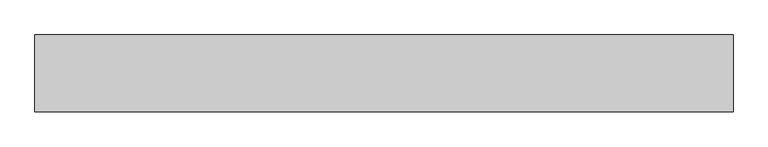
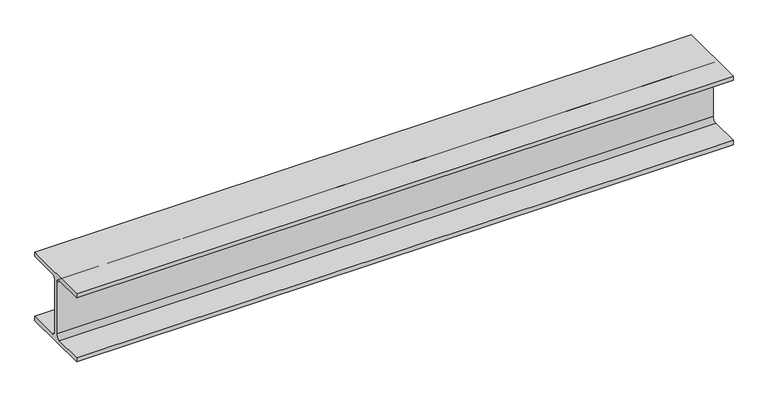
"""IFC4 building model written with IfcOpenShell, lengths in millimetres: beam geometry, 0912_Steel Framing_H-KSD3502 : H_SB_ASB_H-200x200x8x12."""

from ifc_helpers import new_model, si_unit, point, frame, frame_2d, origin, place, context, project, spatial, polyline, circle_curve, trimmed, segment, composite_curve, outline, extrude, source, transform, mapped, element, save


def beam_7ef1a012(model_context):
    return source(origin(), model_context, "Body", "SweptSolid", [
        extrude(outline(composite_curve([segment(polyline([(100.0, -88.0), (100.0, -100.0), (-100.0, -100.0), (-100.0, -88.0), (-17.0, -88.0)]), True, "CONTINUOUS"), segment(trimmed(circle_curve(frame_2d((-17.0, -75.0)), 13.0), [point((-17.0, -88.0))], [point((-4.0, -75.0))], True, "CARTESIAN"), True, "CONTINUOUS"), segment(polyline([(-4.0, -75.0), (-4.0, 75.0)]), True, "CONTINUOUS"), segment(trimmed(circle_curve(frame_2d((-17.0, 75.0)), 13.0), [point((-4.0, 75.0))], [point((-17.0, 88.0))], True, "CARTESIAN"), True, "CONTINUOUS"), segment(polyline([(-17.0, 88.0), (-100.0, 88.0), (-100.0, 100.0), (100.0, 100.0), (100.0, 88.0), (17.0, 88.0)]), True, "CONTINUOUS"), segment(trimmed(circle_curve(frame_2d((17.0, 75.0)), 13.0), [point((17.0, 88.0))], [point((4.0, 75.0))], True, "CARTESIAN"), True, "CONTINUOUS"), segment(polyline([(4.0, 75.0), (4.0, -75.0)]), True, "CONTINUOUS"), segment(trimmed(circle_curve(frame_2d((17.0, -75.0)), 13.0), [point((4.0, -75.0))], [point((17.0, -88.0))], True, "CARTESIAN"), True, "CONTINUOUS"), segment(polyline([(17.0, -88.0), (100.0, -88.0)]), True, "CONTINUOUS")], self_intersect=False)), frame((-785.0333333, 0.0, 0.0), z_axis=(1.0, 0.0, 0.0), x_axis=(0.0, 1.0, 0.0)), (0.0, 0.0, 1.0), 1820.0666667),
    ])


if __name__ == "__main__":
    model = new_model("IFC4")
    model_context = context("Model", 3, world=origin())
    ifc_project = project(units=[si_unit("LENGTHUNIT", "METRE", prefix="MILLI")], contexts=[model_context])
    site = spatial("IfcSite", under=ifc_project)
    building = spatial("IfcBuilding", under=site)
    placement = place(None, origin())
    beam_shape = beam_7ef1a012(model_context)
    element("IfcBeam", 1, ObjectType="0912_Steel Framing_H-KSD3502 : H_SB_ASB_H-200x200x8x12", at=placement, inside=building, context=model_context, shape_type="MappedRepresentation", body=[
        mapped(beam_shape, transform((0.0, 0.0, 0.0), x_axis=(1.0, 0.0, 0.0), y_axis=(0.0, 1.0, 0.0), z_axis=(0.0, 0.0, 1.0))),
    ])
    save(model, "model.ifc")

# Revit data of these elements
# Type "0912_Steel Framing_H-KSD3502 : H_SB_ASB_H-200x200x8x12"
#   H_WM Code_1 = "S01AA002-00001 | Main Steel Structure Fabrication Work | Shelter/Building | Medium Steel - Standard (90KG/M>Weight≥30KG/M) | Material: (   )"
#   H_WM Code_2 = "S03AA028-00001 | Main Steel Structure Erection Work | Shelter/Building | Medium Steel (90KG/M>Weight≥30KG/M) | Material: (   )"
#   H_WM Code_3 = "S01AA010-00001 | Main Steel Structure Fabrication Work | Shelter/Building | Steel Painting/Coating | for Non-Fireproofed Steel Surface, Surface Preparation, Primer, Second & Final Coat | Material: (   )"
#   H_Q'ty Cal Type Tag = "SB-Q2"
#   Width = 20.0 cm
#   Web Thickness = 0.8 cm
#   Web Fillet = 1.3 cm
#   Warping Constant = 141000.0 cm⁶
#   W = 0
#   Torsional Moment of Inertia = 26.2485 cm⁴
#   Section Area = 63.53 cm²
#   Plastic Modulus weak axis = 244.0 cm³
#   Plastic Modulus strong axis = 525.0 cm³
#   Perimeter = 1.16 m²/m
#   Nominal Weight = 49.90 kgf/m
#   Moment of Inertia weak axis = 1600.00 cm⁴
#   Moment of Inertia strong axis = 4720.00 cm⁴
#   Height = 20.0 cm
#   Flange Thickness = 1.2 cm
#   Elastic Modulus weak axis = 160.0 cm³
#   Elastic Modulus strong axis = 472.0 cm³
#   Centroid Vertical = 10.0 cm
#   Centroid Horizontal = 10.0 cm
#   Ix = 47200000
#   Length [instance default] = 1.5240 m
#   Zx = 525000
#   b = 0.2000 m
#   h = 0.2000 m
#   r = 0.0130 m
#   s = 0.0080 m
#   t = 0.0120 m
#   A = 0.006353 m²
#   Structural Material [instance default] = Steel, 45-345
#   Assembly Code = ""
# Element 1 (IfcBeam, "0912_Steel Framing_H-KSD3502 : H_SB_ASB_H-200x200x8x12")
#   Structural Material = none
# Materials
#   "Steel, 45-345": class "Metal", colour RGB 189 187 185, transparency 0, Description = "Steel 345 MPa", Cost = 0
